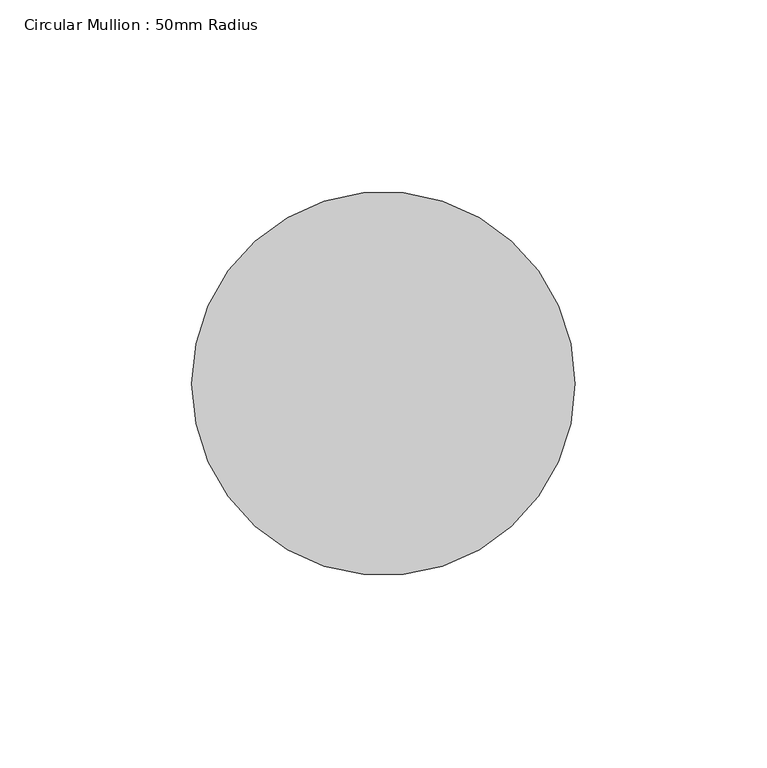
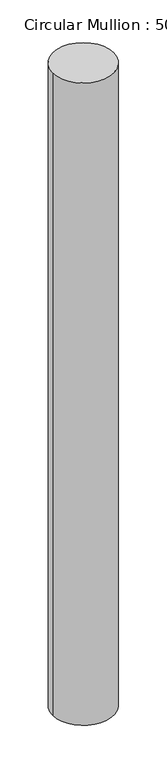
"""IFC4 building model written with IfcOpenShell, lengths in millimetres: member geometry, Circular Mullion : 50mm Radius."""

from ifc_helpers import new_model, si_unit, point, frame, origin, origin_2d, place, context, project, spatial, circle_curve, trimmed, segment, composite_curve, outline, extrude, source, transform, mapped, element, save


def circular_mullion_50mm_radius_57c6cbdf(model_context):
    return source(origin(), model_context, "Body", "SweptSolid", [
        extrude(outline(composite_curve([segment(trimmed(circle_curve(origin_2d(), 50.0), [point((50.0, 0.0))], [point((-50.0, 0.0))], False, "CARTESIAN"), True, "CONTINUOUS"), segment(trimmed(circle_curve(origin_2d(), 50.0), [point((-50.0, 0.0))], [point((50.0, 0.0))], False, "CARTESIAN"), True, "CONTINUOUS")], self_intersect=False)), frame((0.0, 0.0, -1113.724694), z_axis=(0.0, 0.0, 1.0), x_axis=(1.0, 0.0, 0.0)), (0.0, 0.0, 1.0), 1113.724694),
    ])


if __name__ == "__main__":
    model = new_model("IFC4")
    model_context = context("Model", 3, world=origin())
    ifc_project = project(units=[si_unit("LENGTHUNIT", "METRE", prefix="MILLI")], contexts=[model_context])
    site = spatial("IfcSite", under=ifc_project)
    building = spatial("IfcBuilding", under=site)
    placement = place(None, origin())
    circular_mullion_50mm_radius_shape = circular_mullion_50mm_radius_57c6cbdf(model_context)
    element("IfcMember", 1, ObjectType="Circular Mullion : 50mm Radius", at=placement, inside=building, context=model_context, shape_type="MappedRepresentation", body=[
        mapped(circular_mullion_50mm_radius_shape, transform((0.0, 0.0, 0.0), x_axis=(1.0, 0.0, 0.0), y_axis=(0.0, 1.0, 0.0), z_axis=(0.0, 0.0, 1.0))),
    ])
    save(model, "model.ifc")

# Revit data of these elements
# Type "Circular Mullion : 50mm Radius"
#   built-in parameter 1007350 = 0.164042 (stored number, unit not read)
# Element 1 (IfcMember, "Circular Mullion : 50mm Radius")
#   Materials on its faces: "Aluminium"
# Materials
#   "Aluminium": class "Metal", colour RGB 247 247 247, transparency 0, Description = "Aluminium 6061", Cost = 0
